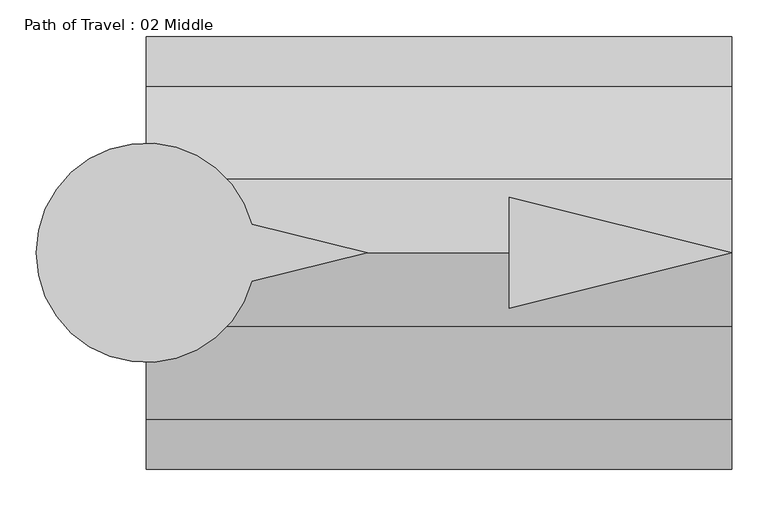
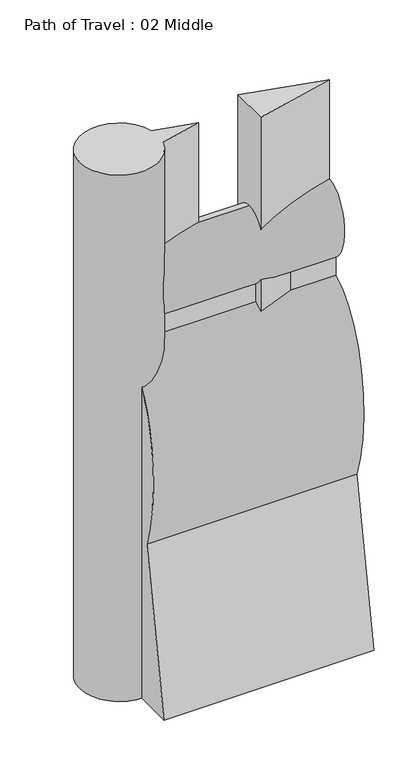
"""IFC4 building model written with IfcOpenShell, lengths in millimetres: proxy geometry, Path of Travel : 02 Middle."""

import ifcopenshell
import ifcopenshell.guid

model = None  # the IFC model being written
_history = None  # IfcOwnerHistory: only IFC2X3 demands one
_inside = {}  # id of a spatial element -> (the spatial element, [elements in it])
_under = {}  # id of a project, library or spatial element -> (it, [spatial elements below it])
_declared = {}  # id of a project -> (the project, [libraries it declares])
_typed = {}  # id of a type object -> (the type object, [elements of that type])
_made_of = {}  # id of a material, layer set ... -> (it, [elements and type objects made of it])


def new_model(schema):
    """Start an empty IFC model of exactly this schema.

    Asked for "IFC4X3", IfcOpenShell would pick the latest addendum, in which some entities
    have other attributes; the version numbers below select the first issue.
    IFC2X3 requires an IfcOwnerHistory on every rooted entity: one is made here for all.
    """
    global model, _history
    if schema == "IFC4X3":
        model = ifcopenshell.file(schema_version=(4, 3, 0, 0))
    else:
        model = ifcopenshell.file(schema=schema)
    _inside.clear()
    _under.clear()
    _declared.clear()
    _typed.clear()
    _made_of.clear()
    _history = None
    if model.schema == "IFC2X3":
        org = make("IfcOrganization", Name="unknown")
        user = make(
            "IfcPersonAndOrganization",
            ThePerson=make("IfcPerson", FamilyName="unknown"),
            TheOrganization=org,
        )
        app = make(
            "IfcApplication",
            ApplicationDeveloper=org,
            Version="unknown",
            ApplicationFullName="unknown",
            ApplicationIdentifier="unknown",
        )
        _history = make(
            "IfcOwnerHistory",
            OwningUser=user,
            OwningApplication=app,
            ChangeAction="ADDED",
            CreationDate=0,
        )
    return model


def make(cls, **values):
    """One entity of the class cls with the attributes given. An attribute that is None is left unset."""
    return model.create_entity(
        cls, **{name: value for name, value in values.items() if value is not None}
    )


def rooted(cls, **values):
    """An entity with a GlobalId (a new one), such as an element, a storey or a relation."""
    return make(cls, GlobalId=ifcopenshell.guid.new(), OwnerHistory=_history, **values)


def si_unit(unit_type, name, prefix=None):
    """IfcSIUnit, for example si_unit("LENGTHUNIT", "METRE", prefix="MILLI")."""
    return make("IfcSIUnit", UnitType=unit_type, Prefix=prefix, Name=name)


def assignment(units):
    """IfcUnitAssignment: the units of a project."""
    return None if units is None else make("IfcUnitAssignment", Units=units)


def point(xyz):
    """IfcCartesianPoint."""
    return None if xyz is None else make("IfcCartesianPoint", Coordinates=xyz)


def direction(xyz):
    """IfcDirection."""
    return None if xyz is None else make("IfcDirection", DirectionRatios=xyz)


def frame(location, z_axis=None, x_axis=None):
    """IfcAxis2Placement3D, a coordinate frame: its origin and axes. An axis left out is left unset."""
    return make(
        "IfcAxis2Placement3D",
        Location=point(location),
        Axis=direction(z_axis),
        RefDirection=direction(x_axis),
    )


def frame_2d(location, x_axis=None):
    """IfcAxis2Placement2D, a coordinate frame in the plane: its origin and x axis."""
    return make(
        "IfcAxis2Placement2D", Location=point(location), RefDirection=direction(x_axis)
    )


def origin():
    """The frame at (0, 0, 0) with its axes left unset."""
    return frame((0.0, 0.0, 0.0))


def origin_with_axes():
    """The frame at (0, 0, 0) with the z axis (0, 0, 1) and the x axis (1, 0, 0) written out."""
    return frame((0.0, 0.0, 0.0), z_axis=(0.0, 0.0, 1.0), x_axis=(1.0, 0.0, 0.0))


def place(relative_to, where):
    """IfcLocalPlacement: puts the frame where relative to a parent placement (None: the world)."""
    return make(
        "IfcLocalPlacement", PlacementRelTo=relative_to, RelativePlacement=where
    )


def context(
    kind, dimensions, precision=None, world=None, true_north=None, identifier=None
):
    """IfcGeometricRepresentationContext, for example the 3D "Model" context."""
    return make(
        "IfcGeometricRepresentationContext",
        ContextIdentifier=identifier,
        ContextType=kind,
        CoordinateSpaceDimension=dimensions,
        Precision=precision,
        WorldCoordinateSystem=world,
        TrueNorth=true_north,
    )


def project(units=None, contexts=None):
    """IfcProject with its units and contexts."""
    return rooted(
        "IfcProject",
        Name="project",
        RepresentationContexts=contexts,
        UnitsInContext=assignment(units),
    )


def spatial(cls, under=None, at=None, **own):
    """A site, building, storey or space (cls), placed at a placement, below another one or the project."""
    s = rooted(cls, ObjectPlacement=at, **own)
    if under is not None:
        _under.setdefault(under.id(), (under, []))[1].append(s)
    return s


def polyline(points):
    """IfcPolyline through the points."""
    return make("IfcPolyline", Points=[point(p) for p in points])


def circle_curve(where, radius):
    """IfcCircle in the frame where."""
    return make("IfcCircle", Position=where, Radius=radius)


def ellipse_curve(where, semi_axis1, semi_axis2):
    """IfcEllipse in the frame where."""
    return make(
        "IfcEllipse", Position=where, SemiAxis1=semi_axis1, SemiAxis2=semi_axis2
    )


def trimmed(basis, trim1, trim2, sense, master):
    """IfcTrimmedCurve: the piece of a basis curve between two trims."""
    return make(
        "IfcTrimmedCurve",
        BasisCurve=basis,
        Trim1=trim1,
        Trim2=trim2,
        SenseAgreement=sense,
        MasterRepresentation=master,
    )


def segment(curve, same_sense, transition):
    """IfcCompositeCurveSegment."""
    return make(
        "IfcCompositeCurveSegment",
        Transition=transition,
        SameSense=same_sense,
        ParentCurve=curve,
    )


def composite_curve(segments, self_intersect=None):
    """IfcCompositeCurve: segments joined end to end."""
    return make("IfcCompositeCurve", Segments=segments, SelfIntersect=self_intersect)


def outline(outer, holes=None, kind="AREA"):
    """IfcArbitraryClosedProfileDef: a profile drawn as a closed curve; with holes, ...WithVoids."""
    if holes is None:
        return make("IfcArbitraryClosedProfileDef", ProfileType=kind, OuterCurve=outer)
    return make(
        "IfcArbitraryProfileDefWithVoids",
        ProfileType=kind,
        OuterCurve=outer,
        InnerCurves=holes,
    )


def extrude(swept, where, along, depth):
    """IfcExtrudedAreaSolid: the profile swept, set in the frame where, extruded along a direction by depth."""
    return make(
        "IfcExtrudedAreaSolid",
        SweptArea=swept,
        Position=where,
        ExtrudedDirection=direction(along),
        Depth=depth,
    )


def shape(context_of_items, identifier, shape_type, items):
    """IfcShapeRepresentation: the items that make up one representation, for example the "Body"."""
    return make(
        "IfcShapeRepresentation",
        ContextOfItems=context_of_items,
        RepresentationIdentifier=identifier,
        RepresentationType=shape_type,
        Items=items,
    )


def source(mapping_origin, context_of_items, identifier, shape_type, items):
    """IfcRepresentationMap: a shape defined once, which mapped items show again and again."""
    return make(
        "IfcRepresentationMap",
        MappingOrigin=mapping_origin,
        MappedRepresentation=shape(context_of_items, identifier, shape_type, items),
    )


def transform(
    local_origin,
    x_axis=None,
    y_axis=None,
    z_axis=None,
    scale=None,
    scale2=None,
    scale3=None,
    uniform=True,
):
    """IfcCartesianTransformationOperator3D, or its non-uniform kind. x_axis, y_axis, z_axis: its Axis1, 2, 3."""
    if uniform:
        return make(
            "IfcCartesianTransformationOperator3D",
            Axis1=direction(x_axis),
            Axis2=direction(y_axis),
            LocalOrigin=point(local_origin),
            Scale=scale,
            Axis3=direction(z_axis),
        )
    return make(
        "IfcCartesianTransformationOperator3DnonUniform",
        Axis1=direction(x_axis),
        Axis2=direction(y_axis),
        LocalOrigin=point(local_origin),
        Scale=scale,
        Axis3=direction(z_axis),
        Scale2=scale2,
        Scale3=scale3,
    )


def mapped(mapping_source, mapping_target):
    """IfcMappedItem: shows the shape of a source again, moved by a transform."""
    return make(
        "IfcMappedItem", MappingSource=mapping_source, MappingTarget=mapping_target
    )


def made_of(thing, what):
    """Note that an element or type object is made of a material, layer set ...; save() writes the relation."""
    if what is not None:
        _made_of.setdefault(what.id(), (what, []))[1].append(thing)
    return thing


def element(
    cls,
    number,
    at=None,
    inside=None,
    cuts=None,
    type_object=None,
    material=None,
    context=None,
    identifier="Body",
    shape_type=None,
    held_by="IfcProductDefinitionShape",
    body=None,
    shapes=None,
    **own,
):
    """One element of the class cls, such as IfcWall. Its Tag is "e" and its number.

    at: its placement. inside: the storey or other place that contains it. cuts: it is an
    opening in that element (IfcRelVoidsElement). A single representation is given by context,
    identifier, shape_type and body (its items); several are given by shapes. held_by: the class
    of the entity that holds the representations. save() writes the other relations.
    """
    e = rooted(cls, Tag="e%d" % number, ObjectPlacement=at, **own)
    if body is not None:
        shapes = [shape(context, identifier, shape_type, body)]
    if shapes is not None:
        e.Representation = make(held_by, Representations=shapes)
    if inside is not None:
        _inside.setdefault(inside.id(), (inside, []))[1].append(e)
    if cuts is not None:
        rooted(
            "IfcRelVoidsElement", RelatingBuildingElement=cuts, RelatedOpeningElement=e
        )
    if type_object is not None:
        _typed.setdefault(type_object.id(), (type_object, []))[1].append(e)
    return made_of(e, material)


def aggregate(whole, parts):
    """IfcRelAggregates: a whole, such as a stair, and the parts it consists of."""
    return rooted("IfcRelAggregates", RelatingObject=whole, RelatedObjects=parts)


def save(model, path):
    """Write the relations noted so far, then the file.

    IfcRelAggregates (storeys below a building ...), IfcRelContainedInSpatialStructure (elements
    in a storey), IfcRelDefinesByType, IfcRelAssociatesMaterial and IfcRelDeclares: one each for
    every whole, place, type object, material and project.
    """
    for whole, parts in _under.values():
        aggregate(whole, parts)
    for where, things in _inside.values():
        rooted(
            "IfcRelContainedInSpatialStructure",
            RelatedElements=things,
            RelatingStructure=where,
        )
    for kind, things in _typed.values():
        rooted("IfcRelDefinesByType", RelatedObjects=things, RelatingType=kind)
    for what, things in _made_of.values():
        rooted("IfcRelAssociatesMaterial", RelatedObjects=things, RelatingMaterial=what)
    for by, libraries in _declared.values():
        rooted("IfcRelDeclares", RelatingContext=by, RelatedDefinitions=libraries)
    model.write(path)


def plane_surface(at):
    """IfcPlane: the flat surface through the origin of the frame at, square to its z axis."""
    return make("IfcPlane", Position=at)


def extruded_surface(curve, direction_of_extrusion, depth):
    """IfcSurfaceOfLinearExtrusion: the curve pushed along a direction by depth."""
    return make(
        "IfcSurfaceOfLinearExtrusion",
        SweptCurve=make("IfcArbitraryOpenProfileDef", ProfileType="CURVE", Curve=curve),
        ExtrudedDirection=direction(direction_of_extrusion),
        Depth=depth,
    )


def advanced_brep(points, edges, surfaces, faces):
    """IfcAdvancedBrep: a solid bounded by faces that lie on surfaces and meet in shared edges.

    An edge is (start, end): straight between two places in points (the first is 0);
    or (start, end, curve); or (start, end, curve, False) where it runs against its curve.
    A face is (place in surfaces, loops), or (place, loops, False) where it looks against
    its surface's normal. A loop lists edges by number (the first is 1), with a minus sign
    where the edge is run from its end to its start. The first loop is the outer one.
    """
    corners = [point(p) for p in points]
    vertices = [make("IfcVertexPoint", VertexGeometry=c) for c in corners]
    made = []
    for start, end, *more in edges:
        made.append(
            make(
                "IfcEdgeCurve",
                EdgeStart=vertices[start],
                EdgeEnd=vertices[end],
                EdgeGeometry=more[0] if more else make("IfcPolyline", Points=[corners[start], corners[end]]),
                SameSense=more[1] if len(more) > 1 else True,
            )
        )
    hull = []
    for where, loops, *sense in faces:
        bounds = []
        for j, loop in enumerate(loops):
            ring = [make("IfcOrientedEdge", EdgeElement=made[abs(k) - 1], Orientation=k > 0) for k in loop]
            bounds.append(
                make(
                    "IfcFaceOuterBound" if j == 0 else "IfcFaceBound",
                    Bound=make("IfcEdgeLoop", EdgeList=ring),
                    Orientation=True,
                )
            )
        hull.append(make("IfcAdvancedFace", Bounds=bounds, FaceSurface=surfaces[where], SameSense=sense[0] if sense else True))
    return make("IfcAdvancedBrep", Outer=make("IfcClosedShell", CfsFaces=hull))


def path_of_travel_02_middle_4844d808(model_context):
    return source(origin(), model_context, "Body", "SolidModel", [
        advanced_brep(
        [(227.5554837, 0.0, 1727.2), (227.5554837, 42.9018657, 1436.6534209), (227.5554837, 42.9018657, 1363.4763406), (227.5554837, 184.1186263, 643.4144547), (227.5554837, 297.5699544, 0.0), (227.5554837, 145.6574193, 0.0), (227.5554837, 0.0, 584.2), (227.5554837, -145.6574193, 0.0), (227.5554837, -297.5699544, 0.0), (227.5554837, -184.1186263, 643.4144547), (227.5554837, -42.9018657, 1363.4763406), (227.5554837, -42.9018657, 1436.6534209), (1032.6003735, 0.0, 1727.2), (1032.6003735, -42.9018657, 1436.6534209), (1032.6003735, -42.9018657, 1363.4763406), (1032.6003735, -184.1186263, 643.4144547), (1032.6003735, -297.5699544, 0.0), (1032.6003735, -145.6574193, 0.0), (1032.6003735, 0.0, 584.2), (1032.6003735, 145.6574193, 0.0), (1032.6003735, 297.5699544, 0.0), (1032.6003735, 184.1186263, 643.4144547), (1032.6003735, 42.9018657, 1363.4763406), (1032.6003735, 42.9018657, 1436.6534209)],
        [
            (0, 1, ellipse_curve(frame((227.5554837, 0.0, 1574.8), z_axis=(-1.0, 0.0, 0.0), x_axis=(0.0, 0.0, 1.0)), 152.4, 101.6)),
            (1, 2),
            (2, 3, ellipse_curve(frame((227.5554837, 0.0, 914.4), z_axis=(-1.0, 0.0, 0.0), x_axis=(0.0, 0.0, -1.0)), 457.2, 228.6)),
            (3, 4),
            (4, 5),
            (5, 6),
            (6, 7),
            (7, 8),
            (8, 9),
            (9, 10, ellipse_curve(frame((227.5554837, 0.0, 914.4), z_axis=(-1.0, 0.0, 0.0), x_axis=(0.0, 0.0, -1.0)), 457.2, 228.6)),
            (10, 11),
            (11, 0, ellipse_curve(frame((227.5554837, 0.0, 1574.8), z_axis=(-1.0, 0.0, 0.0), x_axis=(0.0, 0.0, 1.0)), 152.4, 101.6)),
            (12, 13, ellipse_curve(frame((1032.6003735, 0.0, 1574.8), z_axis=(1.0, 0.0, 0.0), x_axis=(0.0, 0.0, 1.0)), 152.4, 101.6)),
            (13, 14),
            (14, 15, ellipse_curve(frame((1032.6003735, 0.0, 914.4), z_axis=(1.0, 0.0, 0.0), x_axis=(0.0, 0.0, -1.0)), 457.2, 228.6)),
            (15, 16),
            (16, 17),
            (17, 18),
            (18, 19),
            (19, 20),
            (20, 21),
            (21, 22, ellipse_curve(frame((1032.6003735, 0.0, 914.4), z_axis=(1.0, 0.0, 0.0), x_axis=(0.0, 0.0, -1.0)), 457.2, 228.6)),
            (22, 23),
            (23, 12, ellipse_curve(frame((1032.6003735, 0.0, 1574.8), z_axis=(1.0, 0.0, 0.0), x_axis=(0.0, 0.0, 1.0)), 152.4, 101.6)),
            (0, 12),
            (23, 1),
            (22, 2),
            (21, 3),
            (20, 4),
            (19, 5),
            (18, 6),
            (17, 7),
            (16, 8),
            (15, 9),
            (14, 10),
            (13, 11),
        ],
        [
            plane_surface(frame((227.5554837, 0.0, 0.0), z_axis=(-1.0, 0.0, 0.0), x_axis=(0.0, 0.0, 1.0))),
            plane_surface(frame((1032.6003735, 0.0, 0.0), z_axis=(1.0, 0.0, 0.0), x_axis=(0.0, 0.0, 1.0))),
            extruded_surface(trimmed(ellipse_curve(frame((1032.6003735, 0.0, 1574.8), z_axis=(-1.0, 0.0, 0.0), x_axis=(0.0, 0.0, 1.0)), 152.4, 101.6), [point((1032.6003735, 0.0, 1727.2))], [point((1032.6003735, 42.9018657, 1436.6534209))], True, "CARTESIAN"), (-805.0448898, 0.0, 0.0), 805.0448898),
            plane_surface(frame((227.5554837, 42.9018657, 1436.6534209), z_axis=(0.0, 1.0, 0.0), x_axis=(1.0, 0.0, 0.0))),
            extruded_surface(trimmed(ellipse_curve(frame((1032.6003735, 0.0, 914.4), z_axis=(-1.0, 0.0, 0.0), x_axis=(0.0, 0.0, -1.0)), 457.2, 228.6), [point((1032.6003735, 42.9018657, 1363.4763406))], [point((1032.6003735, 184.1186263, 643.4144547))], True, "CARTESIAN"), (-805.0448898, 0.0, 0.0), 805.0448898),
            plane_surface(frame((227.5554837, 184.1186263, 643.4144547), z_axis=(0.0, 0.9848077530122078, 0.1736481776669322), x_axis=(1.0, 0.0, 0.0))),
            plane_surface(frame((227.5554837, 297.5699544, 0.0), z_axis=(0.0, 0.0, -1.0), x_axis=(1.0, 0.0, 0.0))),
            plane_surface(frame((227.5554837, 145.6574193, 0.0), z_axis=(0.0, -0.9702957262760199, -0.2419218955995739), x_axis=(1.0, 0.0, 0.0))),
            plane_surface(frame((227.5554837, 0.0, 584.2), z_axis=(0.0, 0.9702957262759961, -0.24192189559966923), x_axis=(1.0, 0.0, 0.0))),
            plane_surface(frame((227.5554837, -145.6574193, 0.0), z_axis=(0.0, 0.0, -1.0), x_axis=(1.0, 0.0, 0.0))),
            plane_surface(frame((227.5554837, -297.5699544, 0.0), z_axis=(0.0, -0.984807753012208, 0.17364817766693066), x_axis=(1.0, 0.0, 0.0))),
            extruded_surface(trimmed(ellipse_curve(frame((1032.6003735, 0.0, 914.4), z_axis=(-1.0, 0.0, 0.0), x_axis=(0.0, 0.0, -1.0)), 457.2, 228.6), [point((1032.6003735, -184.1186263, 643.4144547))], [point((1032.6003735, -42.9018657, 1363.4763406))], True, "CARTESIAN"), (-805.0448898, 0.0, 0.0), 805.0448898),
            plane_surface(frame((227.5554837, -42.9018657, 1363.4763406), z_axis=(0.0, -1.0, 0.0), x_axis=(1.0, 0.0, 0.0))),
            extruded_surface(trimmed(ellipse_curve(frame((1032.6003735, 0.0, 1574.8), z_axis=(-1.0, 0.0, 0.0), x_axis=(0.0, 0.0, 1.0)), 152.4, 101.6), [point((1032.6003735, -42.9018657, 1436.6534209))], [point((1032.6003735, 0.0, 1727.2))], True, "CARTESIAN"), (-805.0448898, 0.0, 0.0), 805.0448898),
        ],
        [
            (0, [[1, 2, 3, 4, 5, 6, 7, 8, 9, 10, 11, 12]]),
            (1, [[13, 14, 15, 16, 17, 18, 19, 20, 21, 22, 23, 24]]),
            (2, [[-1, 25, -24, 26]]),
            (3, [[-2, -26, -23, 27]]),
            (4, [[-3, -27, -22, 28]]),
            (5, [[-4, -28, -21, 29]]),
            (6, [[-5, -29, -20, 30]]),
            (7, [[-6, -30, -19, 31]]),
            (8, [[-7, -31, -18, 32]]),
            (9, [[-8, -32, -17, 33]]),
            (10, [[-9, -33, -16, 34]]),
            (11, [[-10, -34, -15, 35]]),
            (12, [[-11, -35, -14, 36]]),
            (13, [[-12, -36, -13, -25]]),
        ],
    ),
        extrude(outline(polyline([(726.5952269, 76.2006338), (1032.6003735, 0.0), (726.5952269, -76.2006338), (726.5952269, 76.2006338)])), origin_with_axes(), (0.0, 0.0, 1.0), 2129.5973753),
        extrude(outline(composite_curve([segment(polyline([(372.7837828, 39.4440225), (531.182385, 0.0), (372.7837828, -39.4440225)]), True, "CONTINUOUS"), segment(trimmed(circle_curve(frame_2d((227.2200886, 0.0)), 150.8131956), [point((372.7837828, -39.4440225))], [point((372.7837828, 39.4440225))], False, "CARTESIAN"), True, "CONTINUOUS")], self_intersect=False)), origin_with_axes(), (0.0, 0.0, 1.0), 2129.5973753),
    ])


if __name__ == "__main__":
    model = new_model("IFC4")
    model_context = context("Model", 3, world=origin())
    ifc_project = project(units=[si_unit("LENGTHUNIT", "METRE", prefix="MILLI")], contexts=[model_context])
    site = spatial("IfcSite", under=ifc_project)
    building = spatial("IfcBuilding", under=site)
    placement = place(None, origin())
    path_of_travel_02_middle_shape = path_of_travel_02_middle_4844d808(model_context)
    element("IfcBuildingElementProxy", 1, Name="Path of Travel : 02 Middle", ObjectType="Path of Travel : 02 Middle", at=placement, inside=building, context=model_context, shape_type="MappedRepresentation", body=[
        mapped(path_of_travel_02_middle_shape, transform((0.0, 0.0, 0.0), x_axis=(1.0, 0.0, 0.0), y_axis=(0.0, 1.0, 0.0), z_axis=(0.0, 0.0, 1.0))),
    ])
    save(model, "model.ifc")

# Revit data of these elements
# Type "Path of Travel : 02 Middle"
#   Path of Egress [instance default] = 4' - 0"
#   built-in parameter 1001306 [instance default] = 4 (stored number, unit not read)
#   Dot at Start = no
#   Arrow in Middle = yes
#   Arrow at End = no
#   Egress Path = none
# Element 1 (IfcBuildingElementProxy, "Path of Travel : 02 Middle")
#   Path of Egress = 2' - 7.69468"
#   built-in parameter 1001306 = 2.64122 (stored number, unit not read)
#   Materials on its faces: "Egress Path Solid", "solid"
# Materials
#   "Egress Path Solid": class "Unassigned", colour RGB 255 128 64, transparency 0.75, Comments = "Rendering appearance not upgraded "
#   "solid": class "Generic", colour RGB 120 120 120, transparency 0, Cost = 0
